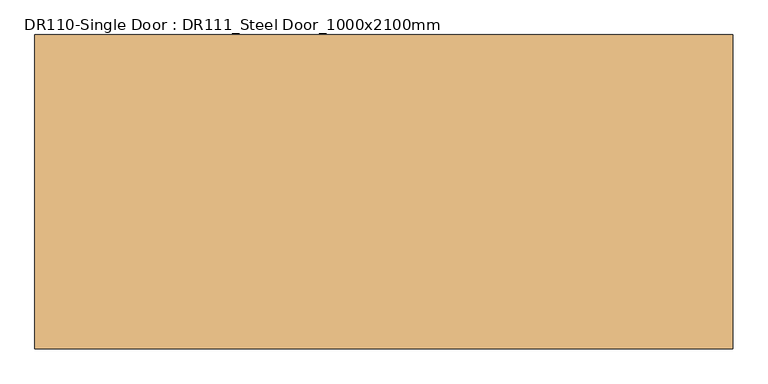
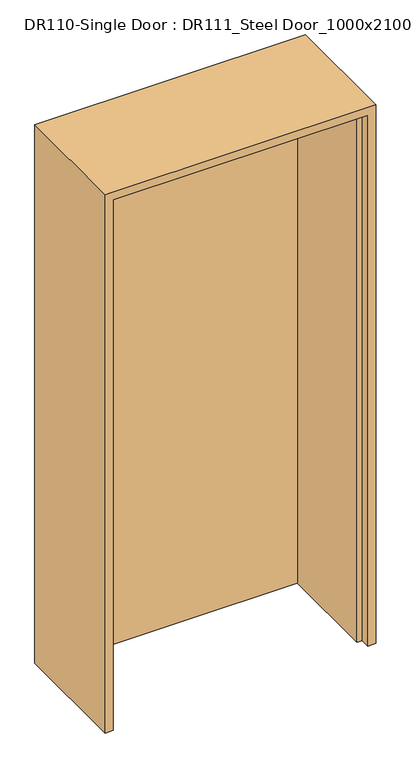
"""IFC4 building model written with IfcOpenShell, lengths in millimetres: door geometry, DR110-Single Door : DR111_Steel Door_1000x2100mm."""

import ifcopenshell
import ifcopenshell.guid

model = None  # the IFC model being written
_history = None  # IfcOwnerHistory: only IFC2X3 demands one
_inside = {}  # id of a spatial element -> (the spatial element, [elements in it])
_under = {}  # id of a project, library or spatial element -> (it, [spatial elements below it])
_declared = {}  # id of a project -> (the project, [libraries it declares])
_typed = {}  # id of a type object -> (the type object, [elements of that type])
_made_of = {}  # id of a material, layer set ... -> (it, [elements and type objects made of it])


def new_model(schema):
    """Start an empty IFC model of exactly this schema.

    Asked for "IFC4X3", IfcOpenShell would pick the latest addendum, in which some entities
    have other attributes; the version numbers below select the first issue.
    IFC2X3 requires an IfcOwnerHistory on every rooted entity: one is made here for all.
    """
    global model, _history
    if schema == "IFC4X3":
        model = ifcopenshell.file(schema_version=(4, 3, 0, 0))
    else:
        model = ifcopenshell.file(schema=schema)
    _inside.clear()
    _under.clear()
    _declared.clear()
    _typed.clear()
    _made_of.clear()
    _history = None
    if model.schema == "IFC2X3":
        org = make("IfcOrganization", Name="unknown")
        user = make(
            "IfcPersonAndOrganization",
            ThePerson=make("IfcPerson", FamilyName="unknown"),
            TheOrganization=org,
        )
        app = make(
            "IfcApplication",
            ApplicationDeveloper=org,
            Version="unknown",
            ApplicationFullName="unknown",
            ApplicationIdentifier="unknown",
        )
        _history = make(
            "IfcOwnerHistory",
            OwningUser=user,
            OwningApplication=app,
            ChangeAction="ADDED",
            CreationDate=0,
        )
    return model


def make(cls, **values):
    """One entity of the class cls with the attributes given. An attribute that is None is left unset."""
    return model.create_entity(
        cls, **{name: value for name, value in values.items() if value is not None}
    )


def rooted(cls, **values):
    """An entity with a GlobalId (a new one), such as an element, a storey or a relation."""
    return make(cls, GlobalId=ifcopenshell.guid.new(), OwnerHistory=_history, **values)


def si_unit(unit_type, name, prefix=None):
    """IfcSIUnit, for example si_unit("LENGTHUNIT", "METRE", prefix="MILLI")."""
    return make("IfcSIUnit", UnitType=unit_type, Prefix=prefix, Name=name)


def assignment(units):
    """IfcUnitAssignment: the units of a project."""
    return None if units is None else make("IfcUnitAssignment", Units=units)


def point(xyz):
    """IfcCartesianPoint."""
    return None if xyz is None else make("IfcCartesianPoint", Coordinates=xyz)


def direction(xyz):
    """IfcDirection."""
    return None if xyz is None else make("IfcDirection", DirectionRatios=xyz)


def frame(location, z_axis=None, x_axis=None):
    """IfcAxis2Placement3D, a coordinate frame: its origin and axes. An axis left out is left unset."""
    return make(
        "IfcAxis2Placement3D",
        Location=point(location),
        Axis=direction(z_axis),
        RefDirection=direction(x_axis),
    )


def origin():
    """The frame at (0, 0, 0) with its axes left unset."""
    return frame((0.0, 0.0, 0.0))


def origin_with_axes():
    """The frame at (0, 0, 0) with the z axis (0, 0, 1) and the x axis (1, 0, 0) written out."""
    return frame((0.0, 0.0, 0.0), z_axis=(0.0, 0.0, 1.0), x_axis=(1.0, 0.0, 0.0))


def place(relative_to, where):
    """IfcLocalPlacement: puts the frame where relative to a parent placement (None: the world)."""
    return make(
        "IfcLocalPlacement", PlacementRelTo=relative_to, RelativePlacement=where
    )


def context(
    kind, dimensions, precision=None, world=None, true_north=None, identifier=None
):
    """IfcGeometricRepresentationContext, for example the 3D "Model" context."""
    return make(
        "IfcGeometricRepresentationContext",
        ContextIdentifier=identifier,
        ContextType=kind,
        CoordinateSpaceDimension=dimensions,
        Precision=precision,
        WorldCoordinateSystem=world,
        TrueNorth=true_north,
    )


def project(units=None, contexts=None):
    """IfcProject with its units and contexts."""
    return rooted(
        "IfcProject",
        Name="project",
        RepresentationContexts=contexts,
        UnitsInContext=assignment(units),
    )


def spatial(cls, under=None, at=None, **own):
    """A site, building, storey or space (cls), placed at a placement, below another one or the project."""
    s = rooted(cls, ObjectPlacement=at, **own)
    if under is not None:
        _under.setdefault(under.id(), (under, []))[1].append(s)
    return s


def polyline(points):
    """IfcPolyline through the points."""
    return make("IfcPolyline", Points=[point(p) for p in points])


def outline(outer, holes=None, kind="AREA"):
    """IfcArbitraryClosedProfileDef: a profile drawn as a closed curve; with holes, ...WithVoids."""
    if holes is None:
        return make("IfcArbitraryClosedProfileDef", ProfileType=kind, OuterCurve=outer)
    return make(
        "IfcArbitraryProfileDefWithVoids",
        ProfileType=kind,
        OuterCurve=outer,
        InnerCurves=holes,
    )


def extrude(swept, where, along, depth):
    """IfcExtrudedAreaSolid: the profile swept, set in the frame where, extruded along a direction by depth."""
    return make(
        "IfcExtrudedAreaSolid",
        SweptArea=swept,
        Position=where,
        ExtrudedDirection=direction(along),
        Depth=depth,
    )


def faces_of(points, faces, orient=None, outer=None):
    """IfcFace entities. A face is a list of loops; a loop is a list of indices into points, from 0.

    orient and outer hold one flag for each loop. By default every Orientation is true, the
    first loop of a face is its IfcFaceOuterBound and the others are IfcFaceBound.
    """
    made = []
    for i, loops in enumerate(faces):
        bounds = []
        for j, loop in enumerate(loops):
            is_outer = j == 0 if outer is None else outer[i][j]
            bounds.append(
                make(
                    "IfcFaceOuterBound" if is_outer else "IfcFaceBound",
                    Bound=make("IfcPolyLoop", Polygon=[points[k] for k in loop]),
                    Orientation=True if orient is None else orient[i][j],
                )
            )
        made.append(make("IfcFace", Bounds=bounds))
    return made


def faceted_brep(points, faces, orient=None, outer=None, voids=None):
    """IfcFacetedBrep: a solid bounded by flat faces; with voids (closed shells), ...WithVoids."""
    shared = [point(p) for p in points]
    hull = make("IfcClosedShell", CfsFaces=faces_of(shared, faces, orient, outer))
    if voids is None:
        return make("IfcFacetedBrep", Outer=hull)
    return make(
        "IfcFacetedBrepWithVoids",
        Outer=hull,
        Voids=[
            make(cls, CfsFaces=faces_of(shared, fs, o, b)) for cls, fs, o, b in voids
        ],
    )


def shape(context_of_items, identifier, shape_type, items):
    """IfcShapeRepresentation: the items that make up one representation, for example the "Body"."""
    return make(
        "IfcShapeRepresentation",
        ContextOfItems=context_of_items,
        RepresentationIdentifier=identifier,
        RepresentationType=shape_type,
        Items=items,
    )


def source(mapping_origin, context_of_items, identifier, shape_type, items):
    """IfcRepresentationMap: a shape defined once, which mapped items show again and again."""
    return make(
        "IfcRepresentationMap",
        MappingOrigin=mapping_origin,
        MappedRepresentation=shape(context_of_items, identifier, shape_type, items),
    )


def transform(
    local_origin,
    x_axis=None,
    y_axis=None,
    z_axis=None,
    scale=None,
    scale2=None,
    scale3=None,
    uniform=True,
):
    """IfcCartesianTransformationOperator3D, or its non-uniform kind. x_axis, y_axis, z_axis: its Axis1, 2, 3."""
    if uniform:
        return make(
            "IfcCartesianTransformationOperator3D",
            Axis1=direction(x_axis),
            Axis2=direction(y_axis),
            LocalOrigin=point(local_origin),
            Scale=scale,
            Axis3=direction(z_axis),
        )
    return make(
        "IfcCartesianTransformationOperator3DnonUniform",
        Axis1=direction(x_axis),
        Axis2=direction(y_axis),
        LocalOrigin=point(local_origin),
        Scale=scale,
        Axis3=direction(z_axis),
        Scale2=scale2,
        Scale3=scale3,
    )


def mapped(mapping_source, mapping_target):
    """IfcMappedItem: shows the shape of a source again, moved by a transform."""
    return make(
        "IfcMappedItem", MappingSource=mapping_source, MappingTarget=mapping_target
    )


def made_of(thing, what):
    """Note that an element or type object is made of a material, layer set ...; save() writes the relation."""
    if what is not None:
        _made_of.setdefault(what.id(), (what, []))[1].append(thing)
    return thing


def element(
    cls,
    number,
    at=None,
    inside=None,
    cuts=None,
    type_object=None,
    material=None,
    context=None,
    identifier="Body",
    shape_type=None,
    held_by="IfcProductDefinitionShape",
    body=None,
    shapes=None,
    **own,
):
    """One element of the class cls, such as IfcWall. Its Tag is "e" and its number.

    at: its placement. inside: the storey or other place that contains it. cuts: it is an
    opening in that element (IfcRelVoidsElement). A single representation is given by context,
    identifier, shape_type and body (its items); several are given by shapes. held_by: the class
    of the entity that holds the representations. save() writes the other relations.
    """
    e = rooted(cls, Tag="e%d" % number, ObjectPlacement=at, **own)
    if body is not None:
        shapes = [shape(context, identifier, shape_type, body)]
    if shapes is not None:
        e.Representation = make(held_by, Representations=shapes)
    if inside is not None:
        _inside.setdefault(inside.id(), (inside, []))[1].append(e)
    if cuts is not None:
        rooted(
            "IfcRelVoidsElement", RelatingBuildingElement=cuts, RelatedOpeningElement=e
        )
    if type_object is not None:
        _typed.setdefault(type_object.id(), (type_object, []))[1].append(e)
    return made_of(e, material)


def aggregate(whole, parts):
    """IfcRelAggregates: a whole, such as a stair, and the parts it consists of."""
    return rooted("IfcRelAggregates", RelatingObject=whole, RelatedObjects=parts)


def save(model, path):
    """Write the relations noted so far, then the file.

    IfcRelAggregates (storeys below a building ...), IfcRelContainedInSpatialStructure (elements
    in a storey), IfcRelDefinesByType, IfcRelAssociatesMaterial and IfcRelDeclares: one each for
    every whole, place, type object, material and project.
    """
    for whole, parts in _under.values():
        aggregate(whole, parts)
    for where, things in _inside.values():
        rooted(
            "IfcRelContainedInSpatialStructure",
            RelatedElements=things,
            RelatingStructure=where,
        )
    for kind, things in _typed.values():
        rooted("IfcRelDefinesByType", RelatedObjects=things, RelatingType=kind)
    for what, things in _made_of.values():
        rooted("IfcRelAssociatesMaterial", RelatedObjects=things, RelatingMaterial=what)
    for by, libraries in _declared.values():
        rooted("IfcRelDeclares", RelatingContext=by, RelatedDefinitions=libraries)
    model.write(path)


def dr110_single_door_dr111_steel_door_1000x2100mm_e52ce95f(model_context):
    return source(origin(), model_context, "Body", "SolidModel", [
        extrude(outline(polyline([(470.0, 225.0), (470.0, 190.0), (-470.0, 190.0), (-470.0, 225.0), (470.0, 225.0)])), origin_with_axes(), (0.0, 0.0, 1.0), 2070.0),
        faceted_brep([(470.0, 225.0, 0.0), (500.0, 225.0, 0.0), (500.0, -225.0, 0.0), (470.0, -225.0, 0.0), (470.0, -190.0, 0.0), (450.0, -190.0, 0.0), (450.0, 190.0, 0.0), (470.0, 190.0, 0.0), (470.0, 225.0, 2070.0), (-470.0, 225.0, 2070.0), (-470.0, 225.0, 0.0), (-500.0, 225.0, 0.0), (-500.0, 225.0, 2100.0), (500.0, 225.0, 2100.0), (500.0, -225.0, 2100.0), (-500.0, -225.0, 2100.0), (-500.0, -225.0, 0.0), (-470.0, -225.0, 0.0), (-470.0, -225.0, 2070.0), (470.0, -225.0, 2070.0), (470.0, -190.0, 2070.0), (-470.0, -190.0, 2070.0), (-470.0, -190.0, 0.0), (-450.0, -190.0, 0.0), (-450.0, -190.0, 2050.0), (450.0, -190.0, 2050.0), (450.0, 190.0, 2050.0), (-450.0, 190.0, 2050.0), (-450.0, 190.0, 0.0), (-470.0, 190.0, 0.0), (-470.0, 190.0, 2070.0), (470.0, 190.0, 2070.0)], [[[0, 1, 2, 3, 4, 5, 6, 7]], [[1, 0, 8, 9, 10, 11, 12, 13]], [[2, 1, 13, 14]], [[3, 2, 14, 15, 16, 17, 18, 19]], [[4, 3, 19, 20]], [[5, 4, 20, 21, 22, 23, 24, 25]], [[6, 5, 25, 26]], [[7, 6, 26, 27, 28, 29, 30, 31]], [[0, 7, 31, 8]], [[9, 30, 29, 10]], [[10, 29, 28, 23, 22, 17, 16, 11]], [[15, 12, 11, 16]], [[21, 18, 17, 22]], [[27, 24, 23, 28]], [[14, 13, 12, 15]], [[20, 19, 18, 21]], [[26, 25, 24, 27]], [[8, 31, 30, 9]]]),
    ])


if __name__ == "__main__":
    model = new_model("IFC4")
    model_context = context("Model", 3, world=origin())
    ifc_project = project(units=[si_unit("LENGTHUNIT", "METRE", prefix="MILLI")], contexts=[model_context])
    site = spatial("IfcSite", under=ifc_project)
    building = spatial("IfcBuilding", under=site)
    placement = place(None, origin())
    dr110_single_door_dr111_steel_door_1000x2100mm_shape = dr110_single_door_dr111_steel_door_1000x2100mm_e52ce95f(model_context)
    element("IfcDoor", 1, ObjectType="DR110-Single Door : DR111_Steel Door_1000x2100mm", at=placement, inside=building, context=model_context, shape_type="MappedRepresentation", body=[
        mapped(dr110_single_door_dr111_steel_door_1000x2100mm_shape, transform((0.0, 0.0, 0.0), x_axis=(1.0, 0.0, 0.0), y_axis=(0.0, 1.0, 0.0), z_axis=(0.0, 0.0, 1.0))),
    ])
    save(model, "model.ifc")

# Revit data of these elements
# Type "DR110-Single Door : DR111_Steel Door_1000x2100mm"
#   Type Mark = "SD"
#   Analytic Construction = "<None>"
#   프레임 투영 외부. = 25 mm
#   프레임 투영 내부. = 25 mm
#   프레임 폭 = 75 mm
#   Height = 2100 mm
#   Width = 1000 mm
#   Define Thermal Properties by = 1
#   문 패널 = SD1 문 패널
#   문 프레임 = A04AQ098-00002_Steel Door_non FP_single
#   Function = (empty or 0)
#   Wall Closure = (empty or 0)
# Element 1 (IfcDoor, "DR110-Single Door : DR111_Steel Door_1000x2100mm")
#   Materials on its faces: "A04AQ098-00002_Steel Door_non FP_single", "SD1 문 패널"
# Materials
#   "SD1 문 패널": class "금속", colour RGB 247 247 247, transparency 0, Description = "STEEL DOOR (1000Wx2100H)"
#   "A04AQ098-00002_Steel Door_non FP_single": class "금속", colour RGB 247 247 247, transparency 0, Description = "Steel Door", W00) Work Master Code = "A04AQ098-00002", W01) Work Master_Lv1 = "Finishing Work", W02) Work Master_Lv2 = "Door & Window Work", W03) Work Master_Spec.1 = "Steel Door w/ Steel Frame", W04) Work Master_Spec.2 = "Fire Protective Rating: N/A, Single Door", W05) Work Master_Spec.3 = "w/ Hardware & Accessories", Cost = 0
